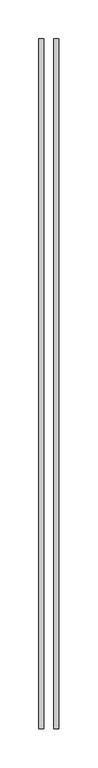
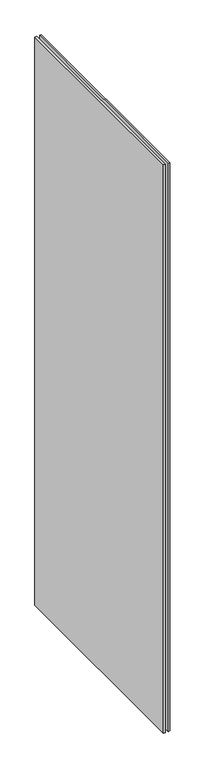
"""IFC4 building model written with IfcOpenShell, lengths in millimetres: proxy geometry, Window glass:Window glass:300352:Window glass:300352 : Window glass:Window glass:300352:300073:Window glass:300352:Window glass:300352 : Window glass:Window glass:300352:300073 : Window glass:Window glass:300352:Window glass:300352 : Window glass:Window glass:300352:300073:4 : Window glass:Window glass:300352:Window glass:300352 : Window glass:Window glass:300352:300073:Window glass:300352:Window glass:300352 : Window glass:Window glass:300352:300073 : Window glass:Window glass:300352:Window glass:300352 : Window glass:Window glass:300352:300073:300061."""

from ifc_helpers import new_model, si_unit, frame, origin, place, context, project, spatial, polyline, outline, extrude, source, transform, mapped, element, save


def generic_models_b6ec3516(model_context):
    return source(origin(), model_context, "Body", "SweptSolid", [
        extrude(outline(polyline([(560292.6367239, -573499.7590038), (560292.6367239, -572612.9375942), (560298.9867239, -572612.9375942), (560298.9867239, -573499.7590038), (560292.6367239, -573499.7590038)])), frame((0.0, 0.0, 55.1405965), z_axis=(0.0, 0.0, 1.0), x_axis=(1.0, 0.0, 0.0)), (0.0, 0.0, 1.0), 2392.531079),
        extrude(outline(polyline([(560311.6867239, -573499.7590038), (560311.6867239, -572612.9375942), (560318.0367239, -572612.9375942), (560318.0367239, -573499.7590038), (560311.6867239, -573499.7590038)])), frame((0.0, 0.0, 55.1405965), z_axis=(0.0, 0.0, 1.0), x_axis=(1.0, 0.0, 0.0)), (0.0, 0.0, 1.0), 2392.531079),
    ])


if __name__ == "__main__":
    model = new_model("IFC4")
    model_context = context("Model", 3, world=origin())
    ifc_project = project(units=[si_unit("LENGTHUNIT", "METRE", prefix="MILLI")], contexts=[model_context])
    site = spatial("IfcSite", under=ifc_project)
    building = spatial("IfcBuilding", under=site)
    placement = place(None, origin())
    generic_models_shape = generic_models_b6ec3516(model_context)
    element("IfcBuildingElementProxy", 1, Name="Window glass:Window glass:300352:Window glass:300352 : Window glass:Window glass:300352:300073:Window glass:300352:Window glass:300352 : Window glass:Window glass:300352:300073 : Window glass:Window glass:300352:Window glass:300352 : Window glass:Window glass:300352:300073:4 : Window glass:Window glass:300352:Window glass:300352 : Window glass:Window glass:300352:300073:Window glass:300352:Window glass:300352 : Window glass:Window glass:300352:300073 : Window glass:Window glass:300352:Window glass:300352 : Window glass:Window glass:300352:300073:300061", ObjectType="Window glass:Window glass:300352:Window glass:300352 : Window glass:Window glass:300352:300073:Window glass:300352:Window glass:300352 : Window glass:Window glass:300352:300073 : Window glass:Window glass:300352:Window glass:300352 : Window glass:Window glass:300352:300073:4 : Window glass:Window glass:300352:Window glass:300352 : Window glass:Window glass:300352:300073:Window glass:300352:Window glass:300352 : Window glass:Window glass:300352:300073 : Window glass:Window glass:300352:Window glass:300352 : Window glass:Window glass:300352:300073:300061", at=placement, inside=building, context=model_context, shape_type="MappedRepresentation", body=[
        mapped(generic_models_shape, transform((0.0, 0.0, 0.0), x_axis=(1.0, 0.0, 0.0), y_axis=(0.0, 1.0, 0.0), z_axis=(0.0, 0.0, 1.0))),
    ])
    save(model, "model.ifc")

# Revit data of these elements
# Type "Window glass:Window glass:300352:Window glass:300352 : Window glass:Window glass:300352:300073:Window glass:300352:Window glass:300352 : Window glass:Window glass:300352:300073 : Window glass:Window glass:300352:Window glass:300352 : Window glass:Window glass:300352:300073:4 : Window glass:Window glass:300352:Window glass:300352 : Window glass:Window glass:300352:300073:Window glass:300352:Window glass:300352 : Window glass:Window glass:300352:300073 : Window glass:Window glass:300352:Window glass:300352 : Window glass:Window glass:300352:300073:300061"
#   NameOverride = "Window glass:Window glass:300352:Window glass:300352 : Window glass:Window glass:300352:300073:Window glass:300352:Window glass:300352 : Window glass:Window glass:300352:300073 : Window glass:Window glass:300352:Window glass:300352 : Window glass:Window glass:300352:300073:300061"
#   ObjectTypeOverride = "Window glass:300352:Window glass:300352 : Window glass:Window glass:300352:300073 : Window glass:Window glass:300352:Window glass:300352 : Window glass:Window glass:300352:300073"
#   Reference = "Window glass"
#   Tag = "300061"
# Element 1 (IfcBuildingElementProxy, "Window glass:Window glass:300352:Window glass:300352 : Window glass:Window glass:300352:300073:Window glass:300352:Window glass:300352 : Window glass:Window glass:300352:300073 : Window glass:Window glass:300352:Window glass:300352 : Window glass:Window glass:300352:300073:4 : Window glass:Window glass:300352:Window glass:300352 : Window glass:Window glass:300352:300073:Window glass:300352:Window glass:300352 : Window glass:Window glass:300352:300073 : Window glass:Window glass:300352:Window glass:300352 : Window glass:Window glass:300352:300073:300061")
#   Materials on its faces: "INSULATED LOW-E GLAZING (SEE ELEVATIONS FOR U-FACTOR, SHGC, & LT)"
# Materials
#   "INSULATED LOW-E GLAZING (SEE ELEVATIONS FOR U-FACTOR, SHGC, & LT)": class "Unassigned", colour RGB 84 171 255, transparency 0, Cost = 0
